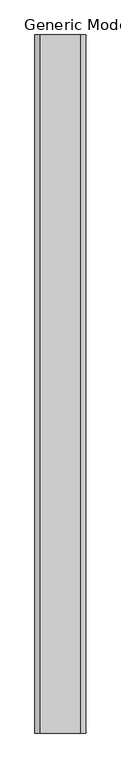
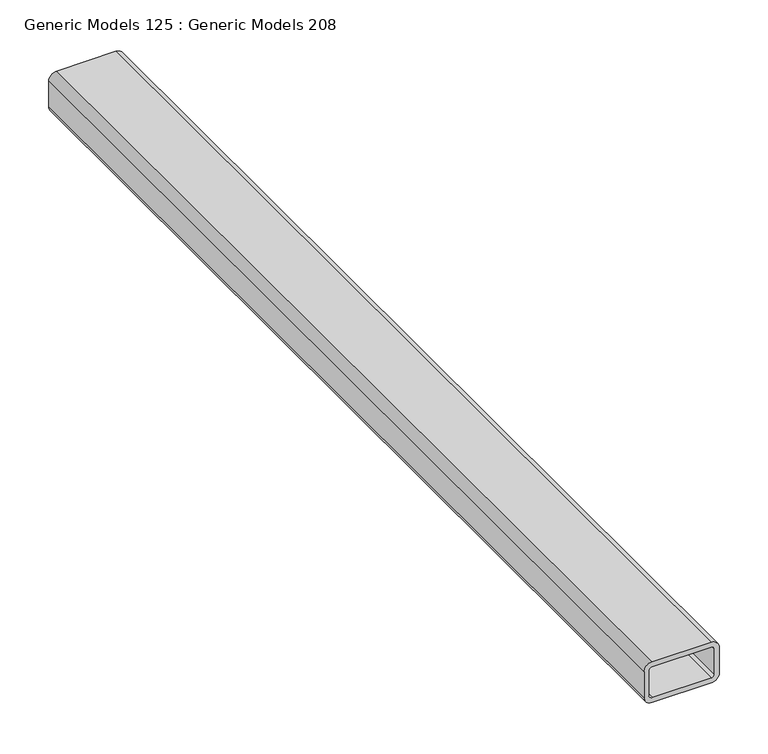
"""IFC4 building model written with IfcOpenShell, lengths in millimetres: proxy geometry, Generic Models 125 : Generic Models 208."""

import ifcopenshell
import ifcopenshell.guid

model = None  # the IFC model being written
_history = None  # IfcOwnerHistory: only IFC2X3 demands one
_inside = {}  # id of a spatial element -> (the spatial element, [elements in it])
_under = {}  # id of a project, library or spatial element -> (it, [spatial elements below it])
_declared = {}  # id of a project -> (the project, [libraries it declares])
_typed = {}  # id of a type object -> (the type object, [elements of that type])
_made_of = {}  # id of a material, layer set ... -> (it, [elements and type objects made of it])


def new_model(schema):
    """Start an empty IFC model of exactly this schema.

    Asked for "IFC4X3", IfcOpenShell would pick the latest addendum, in which some entities
    have other attributes; the version numbers below select the first issue.
    IFC2X3 requires an IfcOwnerHistory on every rooted entity: one is made here for all.
    """
    global model, _history
    if schema == "IFC4X3":
        model = ifcopenshell.file(schema_version=(4, 3, 0, 0))
    else:
        model = ifcopenshell.file(schema=schema)
    _inside.clear()
    _under.clear()
    _declared.clear()
    _typed.clear()
    _made_of.clear()
    _history = None
    if model.schema == "IFC2X3":
        org = make("IfcOrganization", Name="unknown")
        user = make(
            "IfcPersonAndOrganization",
            ThePerson=make("IfcPerson", FamilyName="unknown"),
            TheOrganization=org,
        )
        app = make(
            "IfcApplication",
            ApplicationDeveloper=org,
            Version="unknown",
            ApplicationFullName="unknown",
            ApplicationIdentifier="unknown",
        )
        _history = make(
            "IfcOwnerHistory",
            OwningUser=user,
            OwningApplication=app,
            ChangeAction="ADDED",
            CreationDate=0,
        )
    return model


def make(cls, **values):
    """One entity of the class cls with the attributes given. An attribute that is None is left unset."""
    return model.create_entity(
        cls, **{name: value for name, value in values.items() if value is not None}
    )


def rooted(cls, **values):
    """An entity with a GlobalId (a new one), such as an element, a storey or a relation."""
    return make(cls, GlobalId=ifcopenshell.guid.new(), OwnerHistory=_history, **values)


def si_unit(unit_type, name, prefix=None):
    """IfcSIUnit, for example si_unit("LENGTHUNIT", "METRE", prefix="MILLI")."""
    return make("IfcSIUnit", UnitType=unit_type, Prefix=prefix, Name=name)


def assignment(units):
    """IfcUnitAssignment: the units of a project."""
    return None if units is None else make("IfcUnitAssignment", Units=units)


def point(xyz):
    """IfcCartesianPoint."""
    return None if xyz is None else make("IfcCartesianPoint", Coordinates=xyz)


def direction(xyz):
    """IfcDirection."""
    return None if xyz is None else make("IfcDirection", DirectionRatios=xyz)


def frame(location, z_axis=None, x_axis=None):
    """IfcAxis2Placement3D, a coordinate frame: its origin and axes. An axis left out is left unset."""
    return make(
        "IfcAxis2Placement3D",
        Location=point(location),
        Axis=direction(z_axis),
        RefDirection=direction(x_axis),
    )


def frame_2d(location, x_axis=None):
    """IfcAxis2Placement2D, a coordinate frame in the plane: its origin and x axis."""
    return make(
        "IfcAxis2Placement2D", Location=point(location), RefDirection=direction(x_axis)
    )


def origin():
    """The frame at (0, 0, 0) with its axes left unset."""
    return frame((0.0, 0.0, 0.0))


def place(relative_to, where):
    """IfcLocalPlacement: puts the frame where relative to a parent placement (None: the world)."""
    return make(
        "IfcLocalPlacement", PlacementRelTo=relative_to, RelativePlacement=where
    )


def context(
    kind, dimensions, precision=None, world=None, true_north=None, identifier=None
):
    """IfcGeometricRepresentationContext, for example the 3D "Model" context."""
    return make(
        "IfcGeometricRepresentationContext",
        ContextIdentifier=identifier,
        ContextType=kind,
        CoordinateSpaceDimension=dimensions,
        Precision=precision,
        WorldCoordinateSystem=world,
        TrueNorth=true_north,
    )


def project(units=None, contexts=None):
    """IfcProject with its units and contexts."""
    return rooted(
        "IfcProject",
        Name="project",
        RepresentationContexts=contexts,
        UnitsInContext=assignment(units),
    )


def spatial(cls, under=None, at=None, **own):
    """A site, building, storey or space (cls), placed at a placement, below another one or the project."""
    s = rooted(cls, ObjectPlacement=at, **own)
    if under is not None:
        _under.setdefault(under.id(), (under, []))[1].append(s)
    return s


def polyline(points):
    """IfcPolyline through the points."""
    return make("IfcPolyline", Points=[point(p) for p in points])


def circle_curve(where, radius):
    """IfcCircle in the frame where."""
    return make("IfcCircle", Position=where, Radius=radius)


def trimmed(basis, trim1, trim2, sense, master):
    """IfcTrimmedCurve: the piece of a basis curve between two trims."""
    return make(
        "IfcTrimmedCurve",
        BasisCurve=basis,
        Trim1=trim1,
        Trim2=trim2,
        SenseAgreement=sense,
        MasterRepresentation=master,
    )


def segment(curve, same_sense, transition):
    """IfcCompositeCurveSegment."""
    return make(
        "IfcCompositeCurveSegment",
        Transition=transition,
        SameSense=same_sense,
        ParentCurve=curve,
    )


def composite_curve(segments, self_intersect=None):
    """IfcCompositeCurve: segments joined end to end."""
    return make("IfcCompositeCurve", Segments=segments, SelfIntersect=self_intersect)


def outline(outer, holes=None, kind="AREA"):
    """IfcArbitraryClosedProfileDef: a profile drawn as a closed curve; with holes, ...WithVoids."""
    if holes is None:
        return make("IfcArbitraryClosedProfileDef", ProfileType=kind, OuterCurve=outer)
    return make(
        "IfcArbitraryProfileDefWithVoids",
        ProfileType=kind,
        OuterCurve=outer,
        InnerCurves=holes,
    )


def extrude(swept, where, along, depth):
    """IfcExtrudedAreaSolid: the profile swept, set in the frame where, extruded along a direction by depth."""
    return make(
        "IfcExtrudedAreaSolid",
        SweptArea=swept,
        Position=where,
        ExtrudedDirection=direction(along),
        Depth=depth,
    )


def shape(context_of_items, identifier, shape_type, items):
    """IfcShapeRepresentation: the items that make up one representation, for example the "Body"."""
    return make(
        "IfcShapeRepresentation",
        ContextOfItems=context_of_items,
        RepresentationIdentifier=identifier,
        RepresentationType=shape_type,
        Items=items,
    )


def source(mapping_origin, context_of_items, identifier, shape_type, items):
    """IfcRepresentationMap: a shape defined once, which mapped items show again and again."""
    return make(
        "IfcRepresentationMap",
        MappingOrigin=mapping_origin,
        MappedRepresentation=shape(context_of_items, identifier, shape_type, items),
    )


def transform(
    local_origin,
    x_axis=None,
    y_axis=None,
    z_axis=None,
    scale=None,
    scale2=None,
    scale3=None,
    uniform=True,
):
    """IfcCartesianTransformationOperator3D, or its non-uniform kind. x_axis, y_axis, z_axis: its Axis1, 2, 3."""
    if uniform:
        return make(
            "IfcCartesianTransformationOperator3D",
            Axis1=direction(x_axis),
            Axis2=direction(y_axis),
            LocalOrigin=point(local_origin),
            Scale=scale,
            Axis3=direction(z_axis),
        )
    return make(
        "IfcCartesianTransformationOperator3DnonUniform",
        Axis1=direction(x_axis),
        Axis2=direction(y_axis),
        LocalOrigin=point(local_origin),
        Scale=scale,
        Axis3=direction(z_axis),
        Scale2=scale2,
        Scale3=scale3,
    )


def mapped(mapping_source, mapping_target):
    """IfcMappedItem: shows the shape of a source again, moved by a transform."""
    return make(
        "IfcMappedItem", MappingSource=mapping_source, MappingTarget=mapping_target
    )


def made_of(thing, what):
    """Note that an element or type object is made of a material, layer set ...; save() writes the relation."""
    if what is not None:
        _made_of.setdefault(what.id(), (what, []))[1].append(thing)
    return thing


def element(
    cls,
    number,
    at=None,
    inside=None,
    cuts=None,
    type_object=None,
    material=None,
    context=None,
    identifier="Body",
    shape_type=None,
    held_by="IfcProductDefinitionShape",
    body=None,
    shapes=None,
    **own,
):
    """One element of the class cls, such as IfcWall. Its Tag is "e" and its number.

    at: its placement. inside: the storey or other place that contains it. cuts: it is an
    opening in that element (IfcRelVoidsElement). A single representation is given by context,
    identifier, shape_type and body (its items); several are given by shapes. held_by: the class
    of the entity that holds the representations. save() writes the other relations.
    """
    e = rooted(cls, Tag="e%d" % number, ObjectPlacement=at, **own)
    if body is not None:
        shapes = [shape(context, identifier, shape_type, body)]
    if shapes is not None:
        e.Representation = make(held_by, Representations=shapes)
    if inside is not None:
        _inside.setdefault(inside.id(), (inside, []))[1].append(e)
    if cuts is not None:
        rooted(
            "IfcRelVoidsElement", RelatingBuildingElement=cuts, RelatedOpeningElement=e
        )
    if type_object is not None:
        _typed.setdefault(type_object.id(), (type_object, []))[1].append(e)
    return made_of(e, material)


def aggregate(whole, parts):
    """IfcRelAggregates: a whole, such as a stair, and the parts it consists of."""
    return rooted("IfcRelAggregates", RelatingObject=whole, RelatedObjects=parts)


def save(model, path):
    """Write the relations noted so far, then the file.

    IfcRelAggregates (storeys below a building ...), IfcRelContainedInSpatialStructure (elements
    in a storey), IfcRelDefinesByType, IfcRelAssociatesMaterial and IfcRelDeclares: one each for
    every whole, place, type object, material and project.
    """
    for whole, parts in _under.values():
        aggregate(whole, parts)
    for where, things in _inside.values():
        rooted(
            "IfcRelContainedInSpatialStructure",
            RelatedElements=things,
            RelatingStructure=where,
        )
    for kind, things in _typed.values():
        rooted("IfcRelDefinesByType", RelatedObjects=things, RelatingType=kind)
    for what, things in _made_of.values():
        rooted("IfcRelAssociatesMaterial", RelatedObjects=things, RelatingMaterial=what)
    for by, libraries in _declared.values():
        rooted("IfcRelDeclares", RelatingContext=by, RelatedDefinitions=libraries)
    model.write(path)


def generic_models_125_generic_models_208_d7a22912(model_context):
    return source(origin(), model_context, "Body", "SweptSolid", [
        extrude(outline(composite_curve([segment(trimmed(circle_curve(frame_2d((2230.0862278, 53672.5123648)), 9.4793972), [point((2239.565625, 53672.5123648))], [point((2230.0862278, 53663.0329676))], False, "CARTESIAN"), True, "CONTINUOUS"), segment(polyline([(2230.0862278, 53663.0329676), (2198.2450222, 53663.0329676)]), True, "CONTINUOUS"), segment(trimmed(circle_curve(frame_2d((2198.2450222, 53672.5123648)), 9.4793972), [point((2198.2450222, 53663.0329676))], [point((2188.765625, 53672.5123648))], False, "CARTESIAN"), True, "CONTINUOUS"), segment(polyline([(2188.765625, 53672.5123648), (2188.765625, 53742.4535704)]), True, "CONTINUOUS"), segment(trimmed(circle_curve(frame_2d((2198.2450222, 53742.4535704)), 9.4793972), [point((2188.765625, 53742.4535704))], [point((2198.2450222, 53751.9329676))], False, "CARTESIAN"), True, "CONTINUOUS"), segment(polyline([(2198.2450222, 53751.9329676), (2230.0862278, 53751.9329676)]), True, "CONTINUOUS"), segment(trimmed(circle_curve(frame_2d((2230.0862278, 53742.4535704)), 9.4793972), [point((2230.0862278, 53751.9329676))], [point((2239.565625, 53742.4535704))], False, "CARTESIAN"), True, "CONTINUOUS"), segment(polyline([(2239.565625, 53742.4535704), (2239.565625, 53672.5123648)]), True, "CONTINUOUS")], self_intersect=False), holes=[composite_curve([segment(trimmed(circle_curve(frame_2d((2230.0862278, 53742.4535704)), 3.1293972), [point((2233.215625, 53742.4535704))], [point((2230.0862278, 53745.5829676))], True, "CARTESIAN"), True, "CONTINUOUS"), segment(polyline([(2230.0862278, 53745.5829676), (2198.2450222, 53745.5829676)]), True, "CONTINUOUS"), segment(trimmed(circle_curve(frame_2d((2198.2450222, 53742.4535704)), 3.1293972), [point((2198.2450222, 53745.5829676))], [point((2195.115625, 53742.4535704))], True, "CARTESIAN"), True, "CONTINUOUS"), segment(polyline([(2195.115625, 53742.4535704), (2195.115625, 53672.5123648)]), True, "CONTINUOUS"), segment(trimmed(circle_curve(frame_2d((2198.2450222, 53672.5123648)), 3.1293972), [point((2195.115625, 53672.5123648))], [point((2198.2450222, 53669.3829676))], True, "CARTESIAN"), True, "CONTINUOUS"), segment(polyline([(2198.2450222, 53669.3829676), (2230.0862278, 53669.3829676)]), True, "CONTINUOUS"), segment(trimmed(circle_curve(frame_2d((2230.0862278, 53672.5123648)), 3.1293972), [point((2230.0862278, 53669.3829676))], [point((2233.215625, 53672.5123648))], True, "CARTESIAN"), True, "CONTINUOUS"), segment(polyline([(2233.215625, 53672.5123648), (2233.215625, 53742.4535704)]), True, "CONTINUOUS")], self_intersect=False)]), frame((0.0, -228.7033818, 0.0), z_axis=(0.0, 1.0, 0.0), x_axis=(0.0, 0.0, 1.0)), (0.0, 0.0, 1.0), 1219.2),
    ])


if __name__ == "__main__":
    model = new_model("IFC4")
    model_context = context("Model", 3, world=origin())
    ifc_project = project(units=[si_unit("LENGTHUNIT", "METRE", prefix="MILLI")], contexts=[model_context])
    site = spatial("IfcSite", under=ifc_project)
    building = spatial("IfcBuilding", under=site)
    placement = place(None, origin())
    generic_models_125_generic_models_208_shape = generic_models_125_generic_models_208_d7a22912(model_context)
    element("IfcBuildingElementProxy", 1, Name="Generic Models 125 : Generic Models 208", ObjectType="Generic Models 125 : Generic Models 208", at=placement, inside=building, context=model_context, shape_type="MappedRepresentation", body=[
        mapped(generic_models_125_generic_models_208_shape, transform((0.0, 0.0, 0.0), x_axis=(1.0, 0.0, 0.0), y_axis=(0.0, 1.0, 0.0), z_axis=(0.0, 0.0, 1.0))),
    ])
    save(model, "model.ifc")

# Revit data of these elements
# Element 1 (IfcBuildingElementProxy, "Generic Models 125 : Generic Models 208")
#   Materials on its faces: "TUBE STEEL AS NECESSARY"
# Materials
#   "TUBE STEEL AS NECESSARY": class "Metal", colour RGB 244 244 244, transparency 0, Description = "Aluminum 6061", Cost = 0
